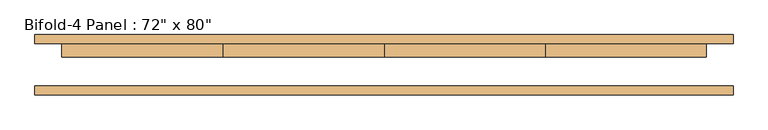
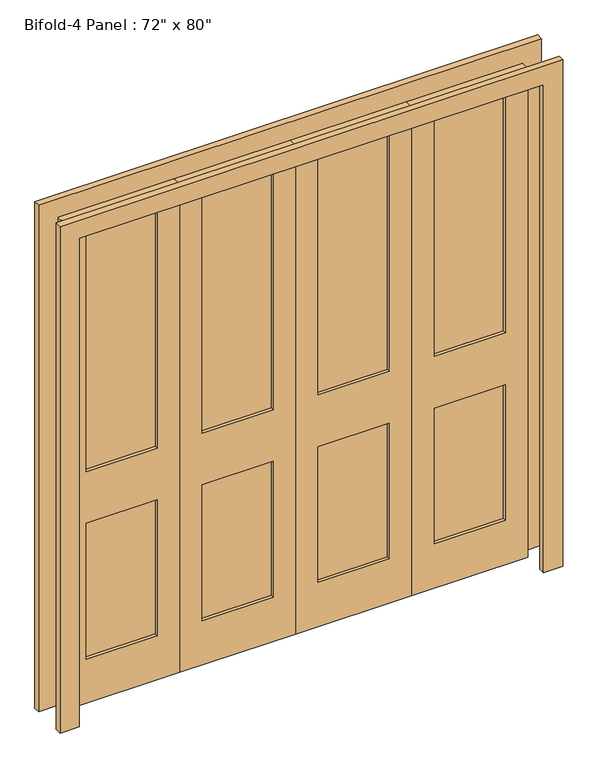
"""IFC4 building model written with IfcOpenShell, lengths in millimetres: door geometry."""

from ifc_helpers import new_model, si_unit, frame, origin, place, context, project, spatial, polyline, outline, extrude, source, transform, mapped, element, save


def door_b3c35402(model_context):
    return source(origin(), model_context, "Body", "SweptSolid", [
        extrude(outline(polyline([(546.1, 47.625), (825.5, 47.625), (825.5, 34.925), (546.1, 34.925), (546.1, 47.625)])), frame((0.0, 0.0, 965.2), z_axis=(0.0, 0.0, 1.0), x_axis=(1.0, 0.0, 0.0)), (0.0, 0.0, 1.0), 984.25),
        extrude(outline(polyline([(546.1, 47.625), (825.5, 47.625), (825.5, 34.925), (546.1, 34.925), (546.1, 47.625)])), frame((0.0, 0.0, 184.15), z_axis=(0.0, 0.0, 1.0), x_axis=(1.0, 0.0, 0.0)), (0.0, 0.0, 1.0), 565.15),
        extrude(outline(polyline([(88.9, 47.625), (368.3, 47.625), (368.3, 34.925), (88.9, 34.925), (88.9, 47.625)])), frame((0.0, 0.0, 965.2), z_axis=(0.0, 0.0, 1.0), x_axis=(1.0, 0.0, 0.0)), (0.0, 0.0, 1.0), 984.25),
        extrude(outline(polyline([(88.9, 47.625), (368.3, 47.625), (368.3, 34.925), (88.9, 34.925), (88.9, 47.625)])), frame((0.0, 0.0, 184.15), z_axis=(0.0, 0.0, 1.0), x_axis=(1.0, 0.0, 0.0)), (0.0, 0.0, 1.0), 565.15),
        extrude(outline(polyline([(-368.3, 47.625), (-88.9, 47.625), (-88.9, 34.925), (-368.3, 34.925), (-368.3, 47.625)])), frame((0.0, 0.0, 184.15), z_axis=(0.0, 0.0, 1.0), x_axis=(1.0, 0.0, 0.0)), (0.0, 0.0, 1.0), 565.15),
        extrude(outline(polyline([(-368.3, 47.625), (-88.9, 47.625), (-88.9, 34.925), (-368.3, 34.925), (-368.3, 47.625)])), frame((0.0, 0.0, 965.2), z_axis=(0.0, 0.0, 1.0), x_axis=(1.0, 0.0, 0.0)), (0.0, 0.0, 1.0), 984.25),
        extrude(outline(polyline([(-825.5, 47.625), (-546.1, 47.625), (-546.1, 34.925), (-825.5, 34.925), (-825.5, 47.625)])), frame((0.0, 0.0, 965.2), z_axis=(0.0, 0.0, 1.0), x_axis=(1.0, 0.0, 0.0)), (0.0, 0.0, 1.0), 984.25),
        extrude(outline(polyline([(-825.5, 47.625), (-546.1, 47.625), (-546.1, 34.925), (-825.5, 34.925), (-825.5, 47.625)])), frame((0.0, 0.0, 184.15), z_axis=(0.0, 0.0, 1.0), x_axis=(1.0, 0.0, 0.0)), (0.0, 0.0, 1.0), 565.15),
        extrude(outline(polyline([(0.0, 990.6), (2108.2, 990.6), (2108.2, -990.6), (0.0, -990.6), (0.0, -914.4), (2032.0, -914.4), (2032.0, 914.4), (0.0, 914.4), (0.0, 990.6)])), frame((0.0, -85.725, 0.0), z_axis=(0.0, 1.0, 0.0), x_axis=(0.0, 0.0, 1.0)), (0.0, 0.0, 1.0), 25.4),
        extrude(outline(polyline([(0.0, 990.6), (2108.2, 990.6), (2108.2, -990.6), (0.0, -990.6), (0.0, -914.4), (2032.0, -914.4), (2032.0, 914.4), (0.0, 914.4), (0.0, 990.6)])), frame((0.0, 60.325, 0.0), z_axis=(0.0, 1.0, 0.0), x_axis=(0.0, 0.0, 1.0)), (0.0, 0.0, 1.0), 25.4),
        extrude(outline(polyline([(0.0, -914.4), (0.0, -457.2), (2032.0, -457.2), (2032.0, -914.4), (0.0, -914.4)]), holes=[polyline([(1949.45, -825.5), (1949.45, -546.1), (965.2, -546.1), (965.2, -825.5), (1949.45, -825.5)]), polyline([(749.3, -825.5), (749.3, -546.1), (184.15, -546.1), (184.15, -825.5), (749.3, -825.5)])]), frame((0.0, 22.225, 0.0), z_axis=(0.0, 1.0, 0.0), x_axis=(0.0, 0.0, 1.0)), (0.0, 0.0, 1.0), 38.1),
        extrude(outline(polyline([(0.0, -457.2), (0.0, 0.0), (2032.0, 0.0), (2032.0, -457.2), (0.0, -457.2)]), holes=[polyline([(1949.45, -368.3), (1949.45, -88.9), (965.2, -88.9), (965.2, -368.3), (1949.45, -368.3)]), polyline([(749.3, -368.3), (749.3, -88.9), (184.15, -88.9), (184.15, -368.3), (749.3, -368.3)])]), frame((0.0, 22.225, 0.0), z_axis=(0.0, 1.0, 0.0), x_axis=(0.0, 0.0, 1.0)), (0.0, 0.0, 1.0), 38.1),
        extrude(outline(polyline([(0.0, 0.0), (0.0, 457.2), (2032.0, 457.2), (2032.0, 0.0), (0.0, 0.0)]), holes=[polyline([(1949.45, 88.9), (1949.45, 368.3), (965.2, 368.3), (965.2, 88.9), (1949.45, 88.9)]), polyline([(749.3, 88.9), (749.3, 368.3), (184.15, 368.3), (184.15, 88.9), (749.3, 88.9)])]), frame((0.0, 22.225, 0.0), z_axis=(0.0, 1.0, 0.0), x_axis=(0.0, 0.0, 1.0)), (0.0, 0.0, 1.0), 38.1),
        extrude(outline(polyline([(0.0, 457.2), (0.0, 914.4), (2032.0, 914.4), (2032.0, 457.2), (0.0, 457.2)]), holes=[polyline([(1949.45, 546.1), (1949.45, 825.5), (965.2, 825.5), (965.2, 546.1), (1949.45, 546.1)]), polyline([(749.3, 546.1), (749.3, 825.5), (184.15, 825.5), (184.15, 546.1), (749.3, 546.1)])]), frame((0.0, 22.225, 0.0), z_axis=(0.0, 1.0, 0.0), x_axis=(0.0, 0.0, 1.0)), (0.0, 0.0, 1.0), 38.1),
    ])


if __name__ == "__main__":
    model = new_model("IFC4")
    model_context = context("Model", 3, world=origin())
    ifc_project = project(units=[si_unit("LENGTHUNIT", "METRE", prefix="MILLI")], contexts=[model_context])
    site = spatial("IfcSite", under=ifc_project)
    building = spatial("IfcBuilding", under=site)
    placement = place(None, origin())
    door_shape = door_b3c35402(model_context)
    element("IfcDoor", 1, ObjectType="Bifold-4 Panel : 72\" x 80\"", at=placement, inside=building, context=model_context, shape_type="MappedRepresentation", body=[
        mapped(door_shape, transform((0.0, 0.0, 0.0), x_axis=(1.0, 0.0, 0.0), y_axis=(0.0, 1.0, 0.0), z_axis=(0.0, 0.0, 1.0))),
    ])
    save(model, "model.ifc")

# Revit data of these elements
# Type "Bifold-4 Panel : 72\" x 80\""
#   Type Mark = "D11"
#   Assembly Code = "C1020"
#   Thickness = 0' - 1 1/2"
#   Height = 6' - 8"
#   Trim Width = 0' - 3"
#   Width = 6' - 0"
#   Door Material = Door - Panel
#   Frame Material = Door - Frame
#   Function = (empty or 0)
#   Description = (empty or 0)
#   Wall Closure = (empty or 0)
# Element 1 (IfcDoor, "Bifold-4 Panel : 72\" x 80\"")
#   Materials on its faces: "Door - Panel", "Door - Frame"
# Materials
#   "Door - Panel": class "Wood", colour RGB 210 159 95, transparency 0, Cost = 0
#   "Door - Frame": class "Miscellaneous", colour RGB 118 70 51, transparency 0, Cost = 0
